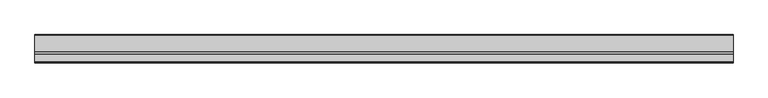
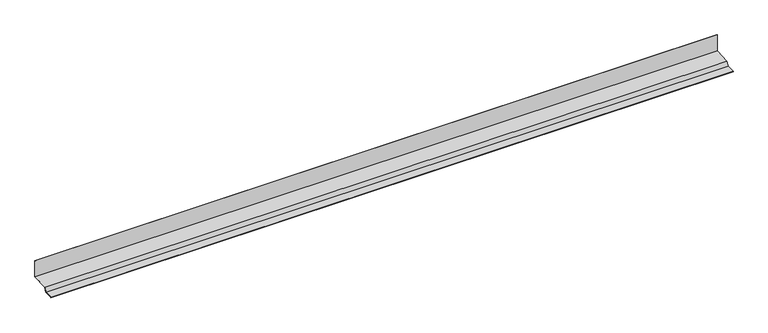
"""IFC4 building model written with IfcOpenShell, lengths in millimetres: proxy geometry, Generic Models 7:Generic Models 1:337419:Generic Models 1:337419 : Generic Models 7:Generic Models 1:337419:9 : Generic Models 7:Generic Models 1:337419:Generic Models 1:337419 : Generic Models 7:Generic Models 1:337419:301336."""

import ifcopenshell
import ifcopenshell.guid

model = None  # the IFC model being written
_history = None  # IfcOwnerHistory: only IFC2X3 demands one
_inside = {}  # id of a spatial element -> (the spatial element, [elements in it])
_under = {}  # id of a project, library or spatial element -> (it, [spatial elements below it])
_declared = {}  # id of a project -> (the project, [libraries it declares])
_typed = {}  # id of a type object -> (the type object, [elements of that type])
_made_of = {}  # id of a material, layer set ... -> (it, [elements and type objects made of it])


def new_model(schema):
    """Start an empty IFC model of exactly this schema.

    Asked for "IFC4X3", IfcOpenShell would pick the latest addendum, in which some entities
    have other attributes; the version numbers below select the first issue.
    IFC2X3 requires an IfcOwnerHistory on every rooted entity: one is made here for all.
    """
    global model, _history
    if schema == "IFC4X3":
        model = ifcopenshell.file(schema_version=(4, 3, 0, 0))
    else:
        model = ifcopenshell.file(schema=schema)
    _inside.clear()
    _under.clear()
    _declared.clear()
    _typed.clear()
    _made_of.clear()
    _history = None
    if model.schema == "IFC2X3":
        org = make("IfcOrganization", Name="unknown")
        user = make(
            "IfcPersonAndOrganization",
            ThePerson=make("IfcPerson", FamilyName="unknown"),
            TheOrganization=org,
        )
        app = make(
            "IfcApplication",
            ApplicationDeveloper=org,
            Version="unknown",
            ApplicationFullName="unknown",
            ApplicationIdentifier="unknown",
        )
        _history = make(
            "IfcOwnerHistory",
            OwningUser=user,
            OwningApplication=app,
            ChangeAction="ADDED",
            CreationDate=0,
        )
    return model


def make(cls, **values):
    """One entity of the class cls with the attributes given. An attribute that is None is left unset."""
    return model.create_entity(
        cls, **{name: value for name, value in values.items() if value is not None}
    )


def rooted(cls, **values):
    """An entity with a GlobalId (a new one), such as an element, a storey or a relation."""
    return make(cls, GlobalId=ifcopenshell.guid.new(), OwnerHistory=_history, **values)


def si_unit(unit_type, name, prefix=None):
    """IfcSIUnit, for example si_unit("LENGTHUNIT", "METRE", prefix="MILLI")."""
    return make("IfcSIUnit", UnitType=unit_type, Prefix=prefix, Name=name)


def assignment(units):
    """IfcUnitAssignment: the units of a project."""
    return None if units is None else make("IfcUnitAssignment", Units=units)


def point(xyz):
    """IfcCartesianPoint."""
    return None if xyz is None else make("IfcCartesianPoint", Coordinates=xyz)


def direction(xyz):
    """IfcDirection."""
    return None if xyz is None else make("IfcDirection", DirectionRatios=xyz)


def frame(location, z_axis=None, x_axis=None):
    """IfcAxis2Placement3D, a coordinate frame: its origin and axes. An axis left out is left unset."""
    return make(
        "IfcAxis2Placement3D",
        Location=point(location),
        Axis=direction(z_axis),
        RefDirection=direction(x_axis),
    )


def origin():
    """The frame at (0, 0, 0) with its axes left unset."""
    return frame((0.0, 0.0, 0.0))


def place(relative_to, where):
    """IfcLocalPlacement: puts the frame where relative to a parent placement (None: the world)."""
    return make(
        "IfcLocalPlacement", PlacementRelTo=relative_to, RelativePlacement=where
    )


def context(
    kind, dimensions, precision=None, world=None, true_north=None, identifier=None
):
    """IfcGeometricRepresentationContext, for example the 3D "Model" context."""
    return make(
        "IfcGeometricRepresentationContext",
        ContextIdentifier=identifier,
        ContextType=kind,
        CoordinateSpaceDimension=dimensions,
        Precision=precision,
        WorldCoordinateSystem=world,
        TrueNorth=true_north,
    )


def project(units=None, contexts=None):
    """IfcProject with its units and contexts."""
    return rooted(
        "IfcProject",
        Name="project",
        RepresentationContexts=contexts,
        UnitsInContext=assignment(units),
    )


def spatial(cls, under=None, at=None, **own):
    """A site, building, storey or space (cls), placed at a placement, below another one or the project."""
    s = rooted(cls, ObjectPlacement=at, **own)
    if under is not None:
        _under.setdefault(under.id(), (under, []))[1].append(s)
    return s


def polyline(points):
    """IfcPolyline through the points."""
    return make("IfcPolyline", Points=[point(p) for p in points])


def outline(outer, holes=None, kind="AREA"):
    """IfcArbitraryClosedProfileDef: a profile drawn as a closed curve; with holes, ...WithVoids."""
    if holes is None:
        return make("IfcArbitraryClosedProfileDef", ProfileType=kind, OuterCurve=outer)
    return make(
        "IfcArbitraryProfileDefWithVoids",
        ProfileType=kind,
        OuterCurve=outer,
        InnerCurves=holes,
    )


def extrude(swept, where, along, depth):
    """IfcExtrudedAreaSolid: the profile swept, set in the frame where, extruded along a direction by depth."""
    return make(
        "IfcExtrudedAreaSolid",
        SweptArea=swept,
        Position=where,
        ExtrudedDirection=direction(along),
        Depth=depth,
    )


def shape(context_of_items, identifier, shape_type, items):
    """IfcShapeRepresentation: the items that make up one representation, for example the "Body"."""
    return make(
        "IfcShapeRepresentation",
        ContextOfItems=context_of_items,
        RepresentationIdentifier=identifier,
        RepresentationType=shape_type,
        Items=items,
    )


def source(mapping_origin, context_of_items, identifier, shape_type, items):
    """IfcRepresentationMap: a shape defined once, which mapped items show again and again."""
    return make(
        "IfcRepresentationMap",
        MappingOrigin=mapping_origin,
        MappedRepresentation=shape(context_of_items, identifier, shape_type, items),
    )


def transform(
    local_origin,
    x_axis=None,
    y_axis=None,
    z_axis=None,
    scale=None,
    scale2=None,
    scale3=None,
    uniform=True,
):
    """IfcCartesianTransformationOperator3D, or its non-uniform kind. x_axis, y_axis, z_axis: its Axis1, 2, 3."""
    if uniform:
        return make(
            "IfcCartesianTransformationOperator3D",
            Axis1=direction(x_axis),
            Axis2=direction(y_axis),
            LocalOrigin=point(local_origin),
            Scale=scale,
            Axis3=direction(z_axis),
        )
    return make(
        "IfcCartesianTransformationOperator3DnonUniform",
        Axis1=direction(x_axis),
        Axis2=direction(y_axis),
        LocalOrigin=point(local_origin),
        Scale=scale,
        Axis3=direction(z_axis),
        Scale2=scale2,
        Scale3=scale3,
    )


def mapped(mapping_source, mapping_target):
    """IfcMappedItem: shows the shape of a source again, moved by a transform."""
    return make(
        "IfcMappedItem", MappingSource=mapping_source, MappingTarget=mapping_target
    )


def made_of(thing, what):
    """Note that an element or type object is made of a material, layer set ...; save() writes the relation."""
    if what is not None:
        _made_of.setdefault(what.id(), (what, []))[1].append(thing)
    return thing


def element(
    cls,
    number,
    at=None,
    inside=None,
    cuts=None,
    type_object=None,
    material=None,
    context=None,
    identifier="Body",
    shape_type=None,
    held_by="IfcProductDefinitionShape",
    body=None,
    shapes=None,
    **own,
):
    """One element of the class cls, such as IfcWall. Its Tag is "e" and its number.

    at: its placement. inside: the storey or other place that contains it. cuts: it is an
    opening in that element (IfcRelVoidsElement). A single representation is given by context,
    identifier, shape_type and body (its items); several are given by shapes. held_by: the class
    of the entity that holds the representations. save() writes the other relations.
    """
    e = rooted(cls, Tag="e%d" % number, ObjectPlacement=at, **own)
    if body is not None:
        shapes = [shape(context, identifier, shape_type, body)]
    if shapes is not None:
        e.Representation = make(held_by, Representations=shapes)
    if inside is not None:
        _inside.setdefault(inside.id(), (inside, []))[1].append(e)
    if cuts is not None:
        rooted(
            "IfcRelVoidsElement", RelatingBuildingElement=cuts, RelatedOpeningElement=e
        )
    if type_object is not None:
        _typed.setdefault(type_object.id(), (type_object, []))[1].append(e)
    return made_of(e, material)


def aggregate(whole, parts):
    """IfcRelAggregates: a whole, such as a stair, and the parts it consists of."""
    return rooted("IfcRelAggregates", RelatingObject=whole, RelatedObjects=parts)


def save(model, path):
    """Write the relations noted so far, then the file.

    IfcRelAggregates (storeys below a building ...), IfcRelContainedInSpatialStructure (elements
    in a storey), IfcRelDefinesByType, IfcRelAssociatesMaterial and IfcRelDeclares: one each for
    every whole, place, type object, material and project.
    """
    for whole, parts in _under.values():
        aggregate(whole, parts)
    for where, things in _inside.values():
        rooted(
            "IfcRelContainedInSpatialStructure",
            RelatedElements=things,
            RelatingStructure=where,
        )
    for kind, things in _typed.values():
        rooted("IfcRelDefinesByType", RelatedObjects=things, RelatingType=kind)
    for what, things in _made_of.values():
        rooted("IfcRelAssociatesMaterial", RelatedObjects=things, RelatingMaterial=what)
    for by, libraries in _declared.values():
        rooted("IfcRelDeclares", RelatingContext=by, RelatedDefinitions=libraries)
    model.write(path)


def generic_models_85619173(model_context):
    return source(origin(), model_context, "Body", "SweptSolid", [
        extrude(outline(polyline([(-568228.2483392, 4481.752118), (-568350.3997175, 4476.6624772), (-568365.1162688, 4448.5291231), (-568426.8080098, 4445.9586339), (-568426.7419213, 4444.3725101), (-568417.5044349, 4444.7574054), (-568417.4713906, 4443.9643435), (-568427.501939, 4443.546404), (-568427.6341159, 4446.7186515), (-568365.6071876, 4449.3031068), (-568350.8906362, 4477.436461), (-568229.0420892, 4482.5134838), (-568229.0420892, 4602.402118), (-568228.2483392, 4602.402118), (-568228.2483392, 4481.752118)])), frame((591306.0367242, 0.0, 0.0), z_axis=(1.0, 0.0, 0.0), x_axis=(0.0, 1.0, 0.0)), (0.0, 0.0, 1.0), 4876.8),
    ])


if __name__ == "__main__":
    model = new_model("IFC4")
    model_context = context("Model", 3, world=origin())
    ifc_project = project(units=[si_unit("LENGTHUNIT", "METRE", prefix="MILLI")], contexts=[model_context])
    site = spatial("IfcSite", under=ifc_project)
    building = spatial("IfcBuilding", under=site)
    placement = place(None, origin())
    generic_models_shape = generic_models_85619173(model_context)
    element("IfcBuildingElementProxy", 1, Name="Generic Models 7:Generic Models 1:337419:Generic Models 1:337419 : Generic Models 7:Generic Models 1:337419:9 : Generic Models 7:Generic Models 1:337419:Generic Models 1:337419 : Generic Models 7:Generic Models 1:337419:301336", ObjectType="Generic Models 7:Generic Models 1:337419:Generic Models 1:337419 : Generic Models 7:Generic Models 1:337419:9 : Generic Models 7:Generic Models 1:337419:Generic Models 1:337419 : Generic Models 7:Generic Models 1:337419:301336", at=placement, inside=building, context=model_context, shape_type="MappedRepresentation", body=[
        mapped(generic_models_shape, transform((0.0, 0.0, 0.0), x_axis=(1.0, 0.0, 0.0), y_axis=(0.0, 1.0, 0.0), z_axis=(0.0, 0.0, 1.0))),
    ])
    save(model, "model.ifc")

# Revit data of these elements
# Type "Generic Models 7:Generic Models 1:337419:Generic Models 1:337419 : Generic Models 7:Generic Models 1:337419:9 : Generic Models 7:Generic Models 1:337419:Generic Models 1:337419 : Generic Models 7:Generic Models 1:337419:301336"
#   NameOverride = "Generic Models 7:Generic Models 1:337419:Generic Models 1:337419 : Generic Models 7:Generic Models 1:337419:301336"
#   ObjectTypeOverride = "Generic Models 1:337419 : Generic Models 7:Generic Models 1:337419"
#   Reference = "Generic Models 1"
#   Tag = "301336"
# Element 1 (IfcBuildingElementProxy, "Generic Models 7:Generic Models 1:337419:Generic Models 1:337419 : Generic Models 7:Generic Models 1:337419:9 : Generic Models 7:Generic Models 1:337419:Generic Models 1:337419 : Generic Models 7:Generic Models 1:337419:301336")
#   Materials on its faces: "PARAPET HIGH EAVE TRIM"
# Materials
#   "PARAPET HIGH EAVE TRIM": class "Unassigned", colour RGB 210 209 208, transparency 0, Cost = 0
